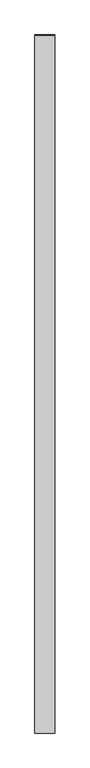
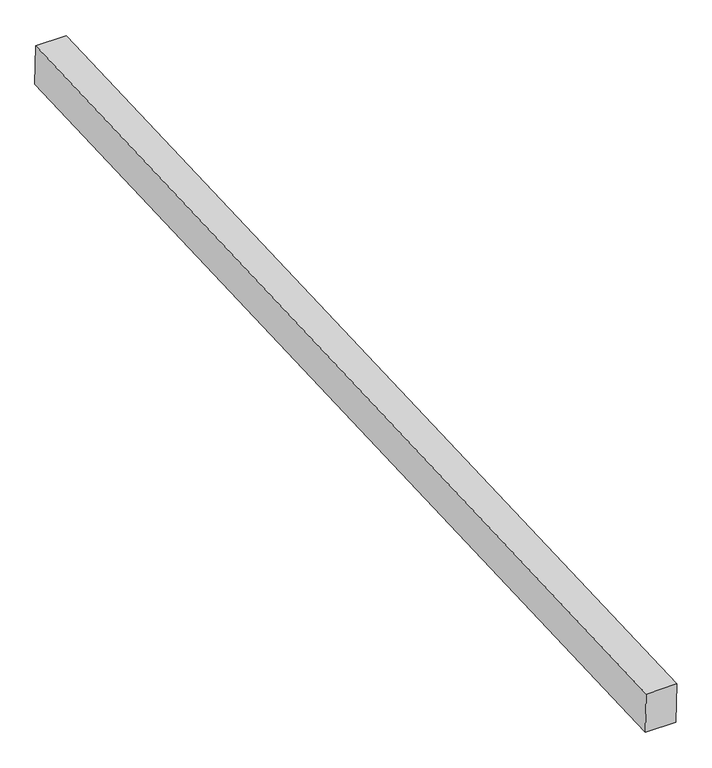
"""IFC4 building model written with IfcOpenShell, lengths in millimetres: proxy geometry, Generic Models 7:Generic Models 1:8:Generic Models 1:8 : Generic Models 7:Generic Models 1:337419:24 : Generic Models 7:Generic Models 1:8:Generic Models 1:8 : Generic Models 7:Generic Models 1:337419:315935."""

from ifc_helpers import new_model, si_unit, frame, origin, place, context, project, spatial, polyline, outline, extrude, source, transform, mapped, element, save


def generic_models_da0d42cf(model_context):
    return source(origin(), model_context, "Body", "SweptSolid", [
        extrude(outline(polyline([(-569809.5331551, 8697.9424054), (-564936.6102609, 8900.9808594), (-564929.0433392, 8710.6308549), (-569801.6025364, 8507.607555), (-569809.5331551, 8697.9424054)])), frame((592439.5117243, 0.0, 0.0), z_axis=(1.0, 0.0, 0.0), x_axis=(0.0, 1.0, 0.0)), (0.0, 0.0, 1.0), 139.7),
    ])


if __name__ == "__main__":
    model = new_model("IFC4")
    model_context = context("Model", 3, world=origin())
    ifc_project = project(units=[si_unit("LENGTHUNIT", "METRE", prefix="MILLI")], contexts=[model_context])
    site = spatial("IfcSite", under=ifc_project)
    building = spatial("IfcBuilding", under=site)
    placement = place(None, origin())
    generic_models_shape = generic_models_da0d42cf(model_context)
    element("IfcBuildingElementProxy", 1, Name="Generic Models 7:Generic Models 1:8:Generic Models 1:8 : Generic Models 7:Generic Models 1:337419:24 : Generic Models 7:Generic Models 1:8:Generic Models 1:8 : Generic Models 7:Generic Models 1:337419:315935", ObjectType="Generic Models 7:Generic Models 1:8:Generic Models 1:8 : Generic Models 7:Generic Models 1:337419:24 : Generic Models 7:Generic Models 1:8:Generic Models 1:8 : Generic Models 7:Generic Models 1:337419:315935", at=placement, inside=building, context=model_context, shape_type="MappedRepresentation", body=[
        mapped(generic_models_shape, transform((0.0, 0.0, 0.0), x_axis=(1.0, 0.0, 0.0), y_axis=(0.0, 1.0, 0.0), z_axis=(0.0, 0.0, 1.0))),
    ])
    save(model, "model.ifc")

# Revit data of these elements
# Type "Generic Models 7:Generic Models 1:8:Generic Models 1:8 : Generic Models 7:Generic Models 1:337419:24 : Generic Models 7:Generic Models 1:8:Generic Models 1:8 : Generic Models 7:Generic Models 1:337419:315935"
#   NameOverride = "Generic Models 7:Generic Models 1:8:Generic Models 1:8 : Generic Models 7:Generic Models 1:337419:315935"
#   ObjectTypeOverride = "Generic Models 1:8 : Generic Models 7:Generic Models 1:337419"
#   Reference = "Generic Models 1"
#   Tag = "315935"
# Element 1 (IfcBuildingElementProxy, "Generic Models 7:Generic Models 1:8:Generic Models 1:8 : Generic Models 7:Generic Models 1:337419:24 : Generic Models 7:Generic Models 1:8:Generic Models 1:8 : Generic Models 7:Generic Models 1:337419:315935")
#   Materials on its faces: "5 1/2\" X 7 1/2\" EXTERIOR GRADE GLULAM BEAMS"
# Materials
#   "5 1/2\" X 7 1/2\" EXTERIOR GRADE GLULAM BEAMS": class "Wood", colour RGB 183 134 68, transparency 0, Keynote = "M06181300.01", Description = "Pinus Echinata", Cost = 0
